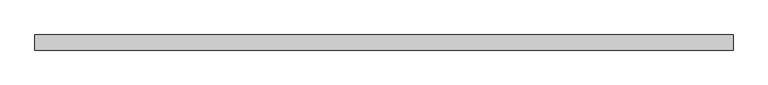
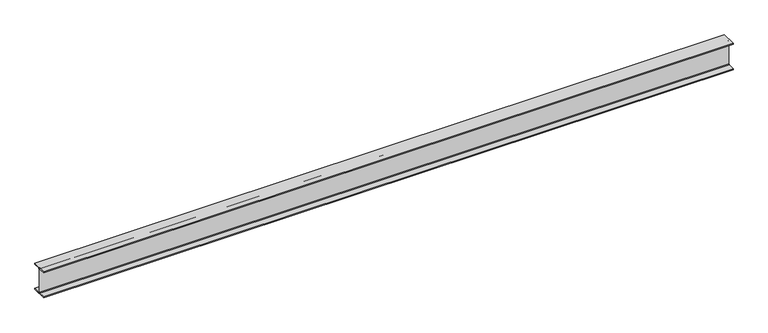
"""IFC4 building model written with IfcOpenShell, lengths in millimetres: beam geometry, Old_Steel Beam_H-KSD3502 : H_SB_ASB_H-300×300x10x15."""

from ifc_helpers import new_model, si_unit, point, frame, frame_2d, origin, place, context, project, spatial, polyline, circle_curve, trimmed, segment, composite_curve, outline, extrude, source, transform, mapped, element, save


def beam_c3343d73(model_context):
    return source(origin(), model_context, "Body", "SweptSolid", [
        extrude(outline(composite_curve([segment(polyline([(82.5, -141.5), (82.5, -151.7), (-82.5, -151.7), (-82.5, -141.5), (-11.9, -141.5)]), True, "CONTINUOUS"), segment(trimmed(circle_curve(frame_2d((-11.9, -132.6)), 8.9), [point((-11.9, -141.5))], [point((-3.0, -132.6))], True, "CARTESIAN"), True, "CONTINUOUS"), segment(polyline([(-3.0, -132.6), (-3.0, 132.6)]), True, "CONTINUOUS"), segment(trimmed(circle_curve(frame_2d((-11.9, 132.6)), 8.9), [point((-3.0, 132.6))], [point((-11.9, 141.5))], True, "CARTESIAN"), True, "CONTINUOUS"), segment(polyline([(-11.9, 141.5), (-82.5, 141.5), (-82.5, 151.7), (82.5, 151.7), (82.5, 141.5), (11.9, 141.5)]), True, "CONTINUOUS"), segment(trimmed(circle_curve(frame_2d((11.9, 132.6)), 8.9), [point((11.9, 141.5))], [point((3.0, 132.6))], True, "CARTESIAN"), True, "CONTINUOUS"), segment(polyline([(3.0, 132.6), (3.0, -132.6)]), True, "CONTINUOUS"), segment(trimmed(circle_curve(frame_2d((11.9, -132.6)), 8.9), [point((3.0, -132.6))], [point((11.9, -141.5))], True, "CARTESIAN"), True, "CONTINUOUS"), segment(polyline([(11.9, -141.5), (82.5, -141.5)]), True, "CONTINUOUS")], self_intersect=False)), frame((-3836.5021141, 0.0, 0.0), z_axis=(1.0, 0.0, 0.0), x_axis=(0.0, 1.0, 0.0)), (0.0, 0.0, 1.0), 7604.5653228),
    ])


if __name__ == "__main__":
    model = new_model("IFC4")
    model_context = context("Model", 3, world=origin())
    ifc_project = project(units=[si_unit("LENGTHUNIT", "METRE", prefix="MILLI")], contexts=[model_context])
    site = spatial("IfcSite", under=ifc_project)
    building = spatial("IfcBuilding", under=site)
    placement = place(None, origin())
    beam_shape = beam_c3343d73(model_context)
    element("IfcBeam", 1, ObjectType="Old_Steel Beam_H-KSD3502 : H_SB_ASB_H-300×300x10x15", at=placement, inside=building, context=model_context, shape_type="MappedRepresentation", body=[
        mapped(beam_shape, transform((0.0, 0.0, 0.0), x_axis=(1.0, 0.0, 0.0), y_axis=(0.0, 1.0, 0.0), z_axis=(0.0, 0.0, 1.0))),
    ])
    save(model, "model.ifc")

# Revit data of these elements
# Type "Old_Steel Beam_H-KSD3502 : H_SB_ASB_H-300×300x10x15"
#   Width = 30.0 cm
#   Web Thickness = 1.0 cm
#   Web Fillet = 1.8 cm
#   Warping Constant = 1370670.0 cm⁶
#   Torsional Moment of Inertia = 77.00 cm⁴
#   Torsional Modulus = 1.0 cm³
#   Section Area = 119.8 cm²
#   Plastic Modulus weak axis = 684.0 cm³
#   Plastic Modulus strong axis = 1500.0 cm³
#   Perimeter = 1.75 m²/m
#   Nominal Weight = 94.00 kgf/m
#   Moment of Inertia weak axis = 6750.00 cm⁴
#   Moment of Inertia strong axis = 20400.00 cm⁴
#   Height = 30.0 cm
#   Flange Thickness = 1.5 cm
#   Elastic Modulus weak axis = 450.0 cm³
#   Elastic Modulus strong axis = 1360.0 cm³
#   Centroid Vertical = 15.0 cm
#   Centroid Horizontal = 15.0 cm
#   Length [instance default] = 1.5240 m
#   Structural Material [instance default] = Steel, 45-345
#   Assembly Code = ""
# Element 1 (IfcBeam, "Old_Steel Beam_H-KSD3502 : H_SB_ASB_H-300×300x10x15")
#   Structural Material = none
# Materials
#   "Steel, 45-345": class "Metal", colour RGB 189 187 185, transparency 0, Description = "Steel 345 MPa", Cost = 0
